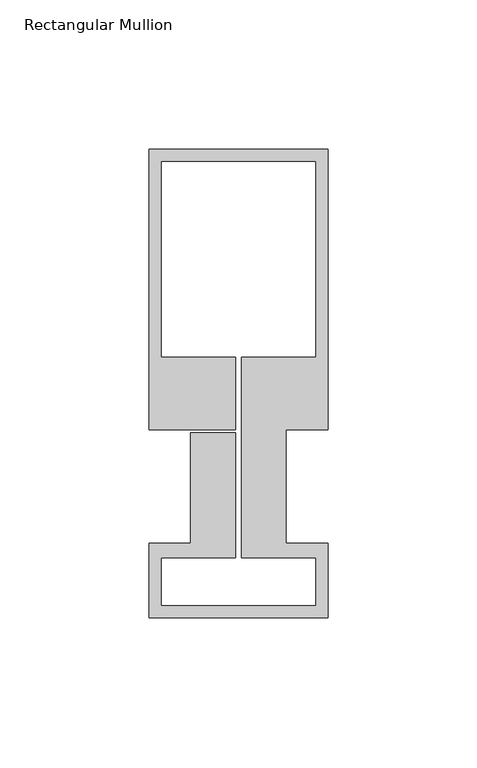
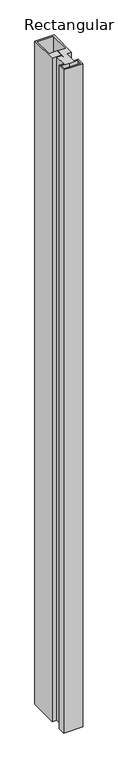
"""IFC4 building model written with IfcOpenShell, lengths in millimetres: member geometry, Rectangular Mullion : Schueco_FWS-60-SI_Mull_CovCap-20mm_Mull-85mm."""

import ifcopenshell
import ifcopenshell.guid

model = None  # the IFC model being written
_history = None  # IfcOwnerHistory: only IFC2X3 demands one
_inside = {}  # id of a spatial element -> (the spatial element, [elements in it])
_under = {}  # id of a project, library or spatial element -> (it, [spatial elements below it])
_declared = {}  # id of a project -> (the project, [libraries it declares])
_typed = {}  # id of a type object -> (the type object, [elements of that type])
_made_of = {}  # id of a material, layer set ... -> (it, [elements and type objects made of it])


def new_model(schema):
    """Start an empty IFC model of exactly this schema.

    Asked for "IFC4X3", IfcOpenShell would pick the latest addendum, in which some entities
    have other attributes; the version numbers below select the first issue.
    IFC2X3 requires an IfcOwnerHistory on every rooted entity: one is made here for all.
    """
    global model, _history
    if schema == "IFC4X3":
        model = ifcopenshell.file(schema_version=(4, 3, 0, 0))
    else:
        model = ifcopenshell.file(schema=schema)
    _inside.clear()
    _under.clear()
    _declared.clear()
    _typed.clear()
    _made_of.clear()
    _history = None
    if model.schema == "IFC2X3":
        org = make("IfcOrganization", Name="unknown")
        user = make(
            "IfcPersonAndOrganization",
            ThePerson=make("IfcPerson", FamilyName="unknown"),
            TheOrganization=org,
        )
        app = make(
            "IfcApplication",
            ApplicationDeveloper=org,
            Version="unknown",
            ApplicationFullName="unknown",
            ApplicationIdentifier="unknown",
        )
        _history = make(
            "IfcOwnerHistory",
            OwningUser=user,
            OwningApplication=app,
            ChangeAction="ADDED",
            CreationDate=0,
        )
    return model


def make(cls, **values):
    """One entity of the class cls with the attributes given. An attribute that is None is left unset."""
    return model.create_entity(
        cls, **{name: value for name, value in values.items() if value is not None}
    )


def rooted(cls, **values):
    """An entity with a GlobalId (a new one), such as an element, a storey or a relation."""
    return make(cls, GlobalId=ifcopenshell.guid.new(), OwnerHistory=_history, **values)


def si_unit(unit_type, name, prefix=None):
    """IfcSIUnit, for example si_unit("LENGTHUNIT", "METRE", prefix="MILLI")."""
    return make("IfcSIUnit", UnitType=unit_type, Prefix=prefix, Name=name)


def assignment(units):
    """IfcUnitAssignment: the units of a project."""
    return None if units is None else make("IfcUnitAssignment", Units=units)


def point(xyz):
    """IfcCartesianPoint."""
    return None if xyz is None else make("IfcCartesianPoint", Coordinates=xyz)


def direction(xyz):
    """IfcDirection."""
    return None if xyz is None else make("IfcDirection", DirectionRatios=xyz)


def frame(location, z_axis=None, x_axis=None):
    """IfcAxis2Placement3D, a coordinate frame: its origin and axes. An axis left out is left unset."""
    return make(
        "IfcAxis2Placement3D",
        Location=point(location),
        Axis=direction(z_axis),
        RefDirection=direction(x_axis),
    )


def origin():
    """The frame at (0, 0, 0) with its axes left unset."""
    return frame((0.0, 0.0, 0.0))


def place(relative_to, where):
    """IfcLocalPlacement: puts the frame where relative to a parent placement (None: the world)."""
    return make(
        "IfcLocalPlacement", PlacementRelTo=relative_to, RelativePlacement=where
    )


def context(
    kind, dimensions, precision=None, world=None, true_north=None, identifier=None
):
    """IfcGeometricRepresentationContext, for example the 3D "Model" context."""
    return make(
        "IfcGeometricRepresentationContext",
        ContextIdentifier=identifier,
        ContextType=kind,
        CoordinateSpaceDimension=dimensions,
        Precision=precision,
        WorldCoordinateSystem=world,
        TrueNorth=true_north,
    )


def project(units=None, contexts=None):
    """IfcProject with its units and contexts."""
    return rooted(
        "IfcProject",
        Name="project",
        RepresentationContexts=contexts,
        UnitsInContext=assignment(units),
    )


def spatial(cls, under=None, at=None, **own):
    """A site, building, storey or space (cls), placed at a placement, below another one or the project."""
    s = rooted(cls, ObjectPlacement=at, **own)
    if under is not None:
        _under.setdefault(under.id(), (under, []))[1].append(s)
    return s


def polyline(points):
    """IfcPolyline through the points."""
    return make("IfcPolyline", Points=[point(p) for p in points])


def outline(outer, holes=None, kind="AREA"):
    """IfcArbitraryClosedProfileDef: a profile drawn as a closed curve; with holes, ...WithVoids."""
    if holes is None:
        return make("IfcArbitraryClosedProfileDef", ProfileType=kind, OuterCurve=outer)
    return make(
        "IfcArbitraryProfileDefWithVoids",
        ProfileType=kind,
        OuterCurve=outer,
        InnerCurves=holes,
    )


def extrude(swept, where, along, depth):
    """IfcExtrudedAreaSolid: the profile swept, set in the frame where, extruded along a direction by depth."""
    return make(
        "IfcExtrudedAreaSolid",
        SweptArea=swept,
        Position=where,
        ExtrudedDirection=direction(along),
        Depth=depth,
    )


def shape(context_of_items, identifier, shape_type, items):
    """IfcShapeRepresentation: the items that make up one representation, for example the "Body"."""
    return make(
        "IfcShapeRepresentation",
        ContextOfItems=context_of_items,
        RepresentationIdentifier=identifier,
        RepresentationType=shape_type,
        Items=items,
    )


def source(mapping_origin, context_of_items, identifier, shape_type, items):
    """IfcRepresentationMap: a shape defined once, which mapped items show again and again."""
    return make(
        "IfcRepresentationMap",
        MappingOrigin=mapping_origin,
        MappedRepresentation=shape(context_of_items, identifier, shape_type, items),
    )


def transform(
    local_origin,
    x_axis=None,
    y_axis=None,
    z_axis=None,
    scale=None,
    scale2=None,
    scale3=None,
    uniform=True,
):
    """IfcCartesianTransformationOperator3D, or its non-uniform kind. x_axis, y_axis, z_axis: its Axis1, 2, 3."""
    if uniform:
        return make(
            "IfcCartesianTransformationOperator3D",
            Axis1=direction(x_axis),
            Axis2=direction(y_axis),
            LocalOrigin=point(local_origin),
            Scale=scale,
            Axis3=direction(z_axis),
        )
    return make(
        "IfcCartesianTransformationOperator3DnonUniform",
        Axis1=direction(x_axis),
        Axis2=direction(y_axis),
        LocalOrigin=point(local_origin),
        Scale=scale,
        Axis3=direction(z_axis),
        Scale2=scale2,
        Scale3=scale3,
    )


def mapped(mapping_source, mapping_target):
    """IfcMappedItem: shows the shape of a source again, moved by a transform."""
    return make(
        "IfcMappedItem", MappingSource=mapping_source, MappingTarget=mapping_target
    )


def made_of(thing, what):
    """Note that an element or type object is made of a material, layer set ...; save() writes the relation."""
    if what is not None:
        _made_of.setdefault(what.id(), (what, []))[1].append(thing)
    return thing


def element(
    cls,
    number,
    at=None,
    inside=None,
    cuts=None,
    type_object=None,
    material=None,
    context=None,
    identifier="Body",
    shape_type=None,
    held_by="IfcProductDefinitionShape",
    body=None,
    shapes=None,
    **own,
):
    """One element of the class cls, such as IfcWall. Its Tag is "e" and its number.

    at: its placement. inside: the storey or other place that contains it. cuts: it is an
    opening in that element (IfcRelVoidsElement). A single representation is given by context,
    identifier, shape_type and body (its items); several are given by shapes. held_by: the class
    of the entity that holds the representations. save() writes the other relations.
    """
    e = rooted(cls, Tag="e%d" % number, ObjectPlacement=at, **own)
    if body is not None:
        shapes = [shape(context, identifier, shape_type, body)]
    if shapes is not None:
        e.Representation = make(held_by, Representations=shapes)
    if inside is not None:
        _inside.setdefault(inside.id(), (inside, []))[1].append(e)
    if cuts is not None:
        rooted(
            "IfcRelVoidsElement", RelatingBuildingElement=cuts, RelatedOpeningElement=e
        )
    if type_object is not None:
        _typed.setdefault(type_object.id(), (type_object, []))[1].append(e)
    return made_of(e, material)


def aggregate(whole, parts):
    """IfcRelAggregates: a whole, such as a stair, and the parts it consists of."""
    return rooted("IfcRelAggregates", RelatingObject=whole, RelatedObjects=parts)


def save(model, path):
    """Write the relations noted so far, then the file.

    IfcRelAggregates (storeys below a building ...), IfcRelContainedInSpatialStructure (elements
    in a storey), IfcRelDefinesByType, IfcRelAssociatesMaterial and IfcRelDeclares: one each for
    every whole, place, type object, material and project.
    """
    for whole, parts in _under.values():
        aggregate(whole, parts)
    for where, things in _inside.values():
        rooted(
            "IfcRelContainedInSpatialStructure",
            RelatedElements=things,
            RelatingStructure=where,
        )
    for kind, things in _typed.values():
        rooted("IfcRelDefinesByType", RelatedObjects=things, RelatingType=kind)
    for what, things in _made_of.values():
        rooted("IfcRelAssociatesMaterial", RelatedObjects=things, RelatingMaterial=what)
    for by, libraries in _declared.values():
        rooted("IfcRelDeclares", RelatingContext=by, RelatedDefinitions=libraries)
    model.write(path)


def rectangular_mullion_58945cea(model_context):
    return source(origin(), model_context, "Body", "SweptSolid", [
        extrude(outline(polyline([(0.0, 132.0), (0.0, 38.0), (-14.0, 38.0), (-14.0, -0.1), (0.0, -0.1), (0.0, -25.0), (-60.0, -25.0), (-60.0, -0.1), (-46.0, -0.1), (-46.0, 37.0), (-31.0, 37.0), (-31.0, -5.0), (-56.0, -5.0), (-56.0, -21.0), (-4.0, -21.0), (-4.0, -5.0), (-29.0, -5.0), (-29.0, 62.3), (-4.0, 62.3), (-4.0, 128.0), (-56.0, 128.0), (-56.0, 62.3), (-31.0, 62.3), (-31.0, 38.0), (-60.0, 38.0), (-60.0, 132.0), (0.0, 132.0)])), frame((0.0, 0.0, -2200.0), z_axis=(0.0, 0.0, 1.0), x_axis=(1.0, 0.0, 0.0)), (0.0, 0.0, 1.0), 2200.0),
    ])


if __name__ == "__main__":
    model = new_model("IFC4")
    model_context = context("Model", 3, world=origin())
    ifc_project = project(units=[si_unit("LENGTHUNIT", "METRE", prefix="MILLI")], contexts=[model_context])
    site = spatial("IfcSite", under=ifc_project)
    building = spatial("IfcBuilding", under=site)
    placement = place(None, origin())
    rectangular_mullion_shape = rectangular_mullion_58945cea(model_context)
    element("IfcMember", 1, ObjectType="Rectangular Mullion : Schueco_FWS-60-SI_Mull_CovCap-20mm_Mull-85mm", at=placement, inside=building, context=model_context, shape_type="MappedRepresentation", body=[
        mapped(rectangular_mullion_shape, transform((0.0, 0.0, 0.0), x_axis=(1.0, 0.0, 0.0), y_axis=(0.0, 1.0, 0.0), z_axis=(0.0, 0.0, 1.0))),
    ])
    save(model, "model.ifc")

# Revit data of these elements
# Type "Rectangular Mullion : Schueco_FWS-60-SI_Mull_CovCap-20mm_Mull-85mm"
#   Model = "FWS 60.SI"
#   Manufacturer = "Schueco International KG"
#   Type Comments = "Mullion"
#   Schueco thermal insulation standard = "Suitable for passive houses"
#   Burglar resistance = "RC 3"
#   Thermal insulation = "to 0.70 W/(m²K)"
#   built-in parameter 1007322 = 0.515092 (stored number, unit not read)
#   built-in parameter 1007321 = 0.0524934 (stored number, unit not read)
#   built-in parameter 1007320 = 0.0524934 (stored number, unit not read)
# Element 1 (IfcMember, "Rectangular Mullion : Schueco_FWS-60-SI_Mull_CovCap-20mm_Mull-85mm")
#   Materials on its faces: "Alu"
# Materials
#   "Alu": class "Glas", colour RGB 140 140 140, transparency 0
